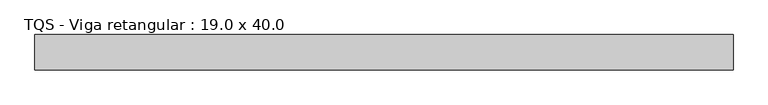
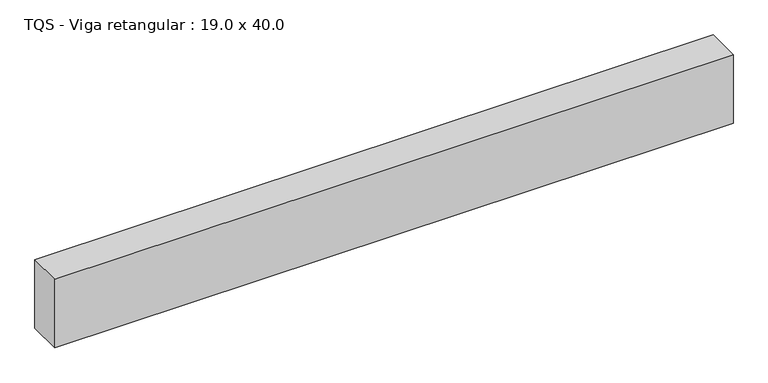
"""IFC4 building model written with IfcOpenShell, lengths in millimetres: beam geometry, TQS - Viga retangular : 19.0 x 40.0."""

from ifc_helpers import new_model, si_unit, frame, origin, place, context, project, spatial, polyline, outline, extrude, source, transform, mapped, element, save


def tqs_viga_retangular_19_0_x_40_0_0a5a2b78(model_context):
    return source(origin(), model_context, "Body", "SweptSolid", [
        extrude(outline(polyline([(1871.5, 95.0), (1871.5, -95.0), (-1871.5, -95.0), (-1871.5, 95.0), (1871.5, 95.0)])), frame((0.0, 0.0, -200.0), z_axis=(0.0, 0.0, 1.0), x_axis=(1.0, 0.0, 0.0)), (0.0, 0.0, 1.0), 400.0),
    ])


if __name__ == "__main__":
    model = new_model("IFC4")
    model_context = context("Model", 3, world=origin())
    ifc_project = project(units=[si_unit("LENGTHUNIT", "METRE", prefix="MILLI")], contexts=[model_context])
    site = spatial("IfcSite", under=ifc_project)
    building = spatial("IfcBuilding", under=site)
    placement = place(None, origin())
    tqs_viga_retangular_19_0_x_40_0_shape = tqs_viga_retangular_19_0_x_40_0_0a5a2b78(model_context)
    element("IfcBeam", 1, ObjectType="TQS - Viga retangular : 19.0 x 40.0", at=placement, inside=building, context=model_context, shape_type="MappedRepresentation", body=[
        mapped(tqs_viga_retangular_19_0_x_40_0_shape, transform((0.0, 0.0, 0.0), x_axis=(1.0, 0.0, 0.0), y_axis=(0.0, 1.0, 0.0), z_axis=(0.0, 0.0, 1.0))),
    ])
    save(model, "model.ifc")

# Revit data of these elements
# Type "TQS - Viga retangular : 19.0 x 40.0"
#   Length [instance default] = 1.524 m
#   b = 0.19 m
#   h = 0.40 m
#   Structural Material [instance default] = none
#   Assembly Code = ""
